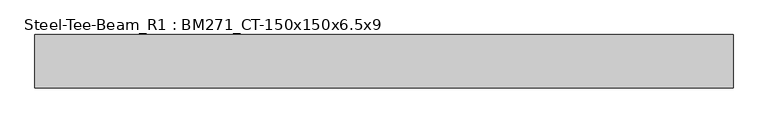
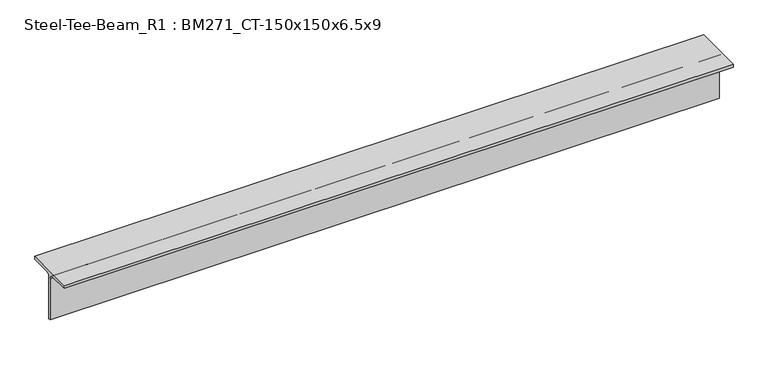
"""IFC4 building model written with IfcOpenShell, lengths in millimetres: member geometry, Steel-Tee-Beam_R1 : BM271_CT-150x150x6.5x9."""

from ifc_helpers import new_model, si_unit, point, frame, frame_2d, origin, place, context, project, spatial, polyline, circle_curve, trimmed, segment, composite_curve, outline, extrude, source, transform, mapped, element, save


def steel_tee_beam_r1_bm271_ct_150x150x6_5x9_ddc2388b(model_context):
    return source(origin(), model_context, "Body", "SweptSolid", [
        extrude(outline(composite_curve([segment(polyline([(-75.0, 75.0), (75.0, 75.0), (75.0, 66.0), (16.25, 66.0)]), True, "CONTINUOUS"), segment(trimmed(circle_curve(frame_2d((16.25, 53.0)), 13.0), [point((16.25, 66.0))], [point((3.25, 53.0))], True, "CARTESIAN"), True, "CONTINUOUS"), segment(polyline([(3.25, 53.0), (3.25, -75.0), (-3.25, -75.0), (-3.25, 53.0)]), True, "CONTINUOUS"), segment(trimmed(circle_curve(frame_2d((-16.25, 53.0)), 13.0), [point((-3.25, 53.0))], [point((-16.25, 66.0))], True, "CARTESIAN"), True, "CONTINUOUS"), segment(polyline([(-16.25, 66.0), (-75.0, 66.0), (-75.0, 75.0)]), True, "CONTINUOUS")], self_intersect=False)), frame((-983.9814396, 0.0, 0.0), z_axis=(1.0, 0.0, 0.0), x_axis=(0.0, 1.0, 0.0)), (0.0, 0.0, 1.0), 1967.9628792),
    ])


if __name__ == "__main__":
    model = new_model("IFC4")
    model_context = context("Model", 3, world=origin())
    ifc_project = project(units=[si_unit("LENGTHUNIT", "METRE", prefix="MILLI")], contexts=[model_context])
    site = spatial("IfcSite", under=ifc_project)
    building = spatial("IfcBuilding", under=site)
    placement = place(None, origin())
    steel_tee_beam_r1_bm271_ct_150x150x6_5x9_shape = steel_tee_beam_r1_bm271_ct_150x150x6_5x9_ddc2388b(model_context)
    element("IfcMember", 1, ObjectType="Steel-Tee-Beam_R1 : BM271_CT-150x150x6.5x9", at=placement, inside=building, context=model_context, shape_type="MappedRepresentation", body=[
        mapped(steel_tee_beam_r1_bm271_ct_150x150x6_5x9_shape, transform((0.0, 0.0, 0.0), x_axis=(1.0, 0.0, 0.0), y_axis=(0.0, 1.0, 0.0), z_axis=(0.0, 0.0, 1.0))),
    ])
    save(model, "model.ifc")

# Revit data of these elements
# Type "Steel-Tee-Beam_R1 : BM271_CT-150x150x6.5x9"
#   Keynote = "CT-150x150x6.5x9"
#   Surface Area = 0.588841 m²/m
#   Section Area = 23.3904 cm²
#   Mass per Unit Length = 18.3614 kg/m
#   Length [instance default] = 1.5240 m
#   bf = 0.1500 m
#   d = 0.1500 m
#   k = 0.0220 m
#   r = 0.0130 m
#   tf = 0.0090 m
#   tw = 0.0065 m
#   hec_material4 [instance default] = none
#   hec_material3 [instance default] = none
#   hec_material2 [instance default] = none
#   hec_material1 [instance default] = none
#   Structural Material [instance default] = Steel, 45-345
#   Assembly Code = ""
# Element 1 (IfcMember, "Steel-Tee-Beam_R1 : BM271_CT-150x150x6.5x9")
#   Structural Material = none
# Materials
#   "Steel, 45-345": class "Metal", colour RGB 189 187 185, transparency 0, Description = "Steel 345 MPa", Cost = 0
